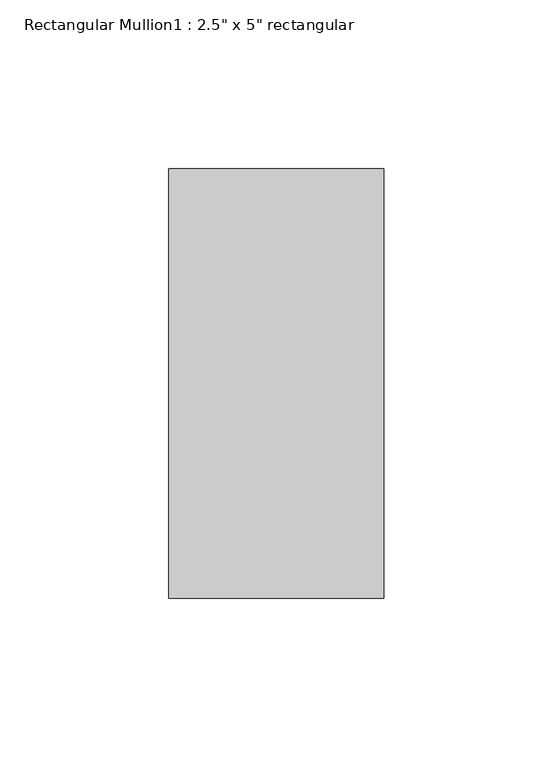
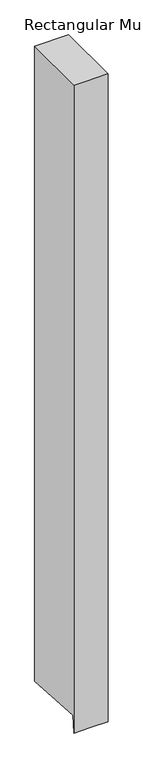
"""IFC4 building model written with IfcOpenShell, lengths in millimetres: member geometry."""

from ifc_helpers import new_model, si_unit, origin, place, context, project, spatial, faceted_brep, source, transform, mapped, element, save


def member_21287d99(model_context):
    return source(origin(), model_context, "Body", "Brep", [
        faceted_brep([(31.75, 63.5, 0.0), (-31.75, 63.5, 0.0), (-31.75, -63.5, 0.0), (31.75, -63.5, 0.0), (31.75, 63.5, -1253.5867756), (0.0, 63.5, -1253.5867756), (-31.75, 63.5, -1253.5867756), (-31.75, -61.1522336, -1244.9455147), (-31.75, -63.5, -1278.8126009), (0.0, -63.5, -1278.8126009), (31.75, -63.5, -1278.8126009), (31.75, -61.1522336, -1244.9455147), (0.0, -61.1522336, -1244.9455147)], [[[0, 1, 2, 3]], [[1, 0, 4, 5, 6]], [[2, 1, 6, 7, 8]], [[3, 2, 8, 9, 10]], [[0, 3, 10, 11, 4]], [[4, 11, 12, 5]], [[11, 10, 9, 12]], [[9, 8, 7, 12]], [[7, 6, 5, 12]]]),
    ])


if __name__ == "__main__":
    model = new_model("IFC4")
    model_context = context("Model", 3, world=origin())
    ifc_project = project(units=[si_unit("LENGTHUNIT", "METRE", prefix="MILLI")], contexts=[model_context])
    site = spatial("IfcSite", under=ifc_project)
    building = spatial("IfcBuilding", under=site)
    placement = place(None, origin())
    member_shape = member_21287d99(model_context)
    element("IfcMember", 1, ObjectType="Rectangular Mullion1 : 2.5\" x 5\" rectangular", at=placement, inside=building, context=model_context, shape_type="MappedRepresentation", body=[
        mapped(member_shape, transform((0.0, 0.0, 0.0), x_axis=(1.0, 0.0, 0.0), y_axis=(0.0, 1.0, 0.0), z_axis=(0.0, 0.0, 1.0))),
    ])
    save(model, "model.ifc")

# Revit data of these elements
# Type "Rectangular Mullion1 : 2.5\" x 5\" rectangular"
#   built-in parameter 1007304 = 0.416667 (stored number, unit not read)
#   built-in parameter 1007301 = 0.104167 (stored number, unit not read)
#   built-in parameter 1007300 = 0.104167 (stored number, unit not read)
# Element 1 (IfcMember, "Rectangular Mullion1 : 2.5\" x 5\" rectangular")
#   Materials on its faces: "support-frame"
# Materials
#   "support-frame": class "Unassigned", colour RGB 233 233 233, transparency 0, Cost = 0
